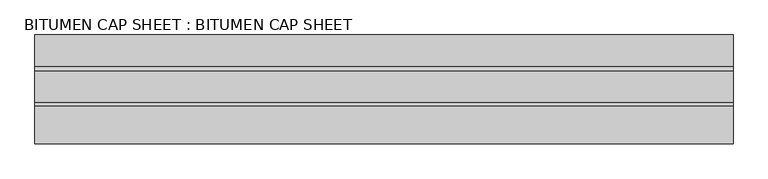
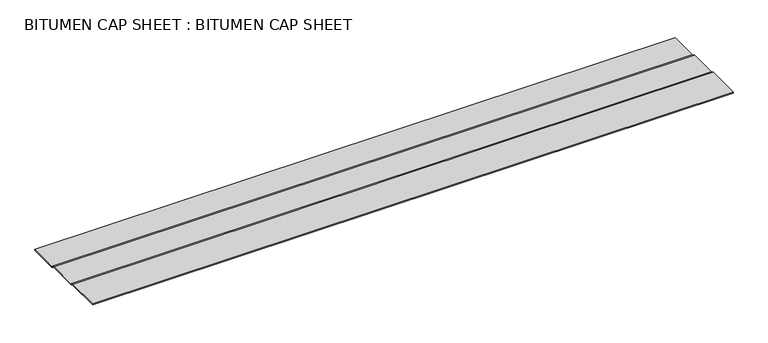
"""IFC4 building model written with IfcOpenShell, lengths in millimetres: proxy geometry, BITUMEN CAP SHEET : BITUMEN CAP SHEET."""

import ifcopenshell
import ifcopenshell.guid

model = None  # the IFC model being written
_history = None  # IfcOwnerHistory: only IFC2X3 demands one
_inside = {}  # id of a spatial element -> (the spatial element, [elements in it])
_under = {}  # id of a project, library or spatial element -> (it, [spatial elements below it])
_declared = {}  # id of a project -> (the project, [libraries it declares])
_typed = {}  # id of a type object -> (the type object, [elements of that type])
_made_of = {}  # id of a material, layer set ... -> (it, [elements and type objects made of it])


def new_model(schema):
    """Start an empty IFC model of exactly this schema.

    Asked for "IFC4X3", IfcOpenShell would pick the latest addendum, in which some entities
    have other attributes; the version numbers below select the first issue.
    IFC2X3 requires an IfcOwnerHistory on every rooted entity: one is made here for all.
    """
    global model, _history
    if schema == "IFC4X3":
        model = ifcopenshell.file(schema_version=(4, 3, 0, 0))
    else:
        model = ifcopenshell.file(schema=schema)
    _inside.clear()
    _under.clear()
    _declared.clear()
    _typed.clear()
    _made_of.clear()
    _history = None
    if model.schema == "IFC2X3":
        org = make("IfcOrganization", Name="unknown")
        user = make(
            "IfcPersonAndOrganization",
            ThePerson=make("IfcPerson", FamilyName="unknown"),
            TheOrganization=org,
        )
        app = make(
            "IfcApplication",
            ApplicationDeveloper=org,
            Version="unknown",
            ApplicationFullName="unknown",
            ApplicationIdentifier="unknown",
        )
        _history = make(
            "IfcOwnerHistory",
            OwningUser=user,
            OwningApplication=app,
            ChangeAction="ADDED",
            CreationDate=0,
        )
    return model


def make(cls, **values):
    """One entity of the class cls with the attributes given. An attribute that is None is left unset."""
    return model.create_entity(
        cls, **{name: value for name, value in values.items() if value is not None}
    )


def rooted(cls, **values):
    """An entity with a GlobalId (a new one), such as an element, a storey or a relation."""
    return make(cls, GlobalId=ifcopenshell.guid.new(), OwnerHistory=_history, **values)


def si_unit(unit_type, name, prefix=None):
    """IfcSIUnit, for example si_unit("LENGTHUNIT", "METRE", prefix="MILLI")."""
    return make("IfcSIUnit", UnitType=unit_type, Prefix=prefix, Name=name)


def assignment(units):
    """IfcUnitAssignment: the units of a project."""
    return None if units is None else make("IfcUnitAssignment", Units=units)


def point(xyz):
    """IfcCartesianPoint."""
    return None if xyz is None else make("IfcCartesianPoint", Coordinates=xyz)


def direction(xyz):
    """IfcDirection."""
    return None if xyz is None else make("IfcDirection", DirectionRatios=xyz)


def frame(location, z_axis=None, x_axis=None):
    """IfcAxis2Placement3D, a coordinate frame: its origin and axes. An axis left out is left unset."""
    return make(
        "IfcAxis2Placement3D",
        Location=point(location),
        Axis=direction(z_axis),
        RefDirection=direction(x_axis),
    )


def origin():
    """The frame at (0, 0, 0) with its axes left unset."""
    return frame((0.0, 0.0, 0.0))


def place(relative_to, where):
    """IfcLocalPlacement: puts the frame where relative to a parent placement (None: the world)."""
    return make(
        "IfcLocalPlacement", PlacementRelTo=relative_to, RelativePlacement=where
    )


def context(
    kind, dimensions, precision=None, world=None, true_north=None, identifier=None
):
    """IfcGeometricRepresentationContext, for example the 3D "Model" context."""
    return make(
        "IfcGeometricRepresentationContext",
        ContextIdentifier=identifier,
        ContextType=kind,
        CoordinateSpaceDimension=dimensions,
        Precision=precision,
        WorldCoordinateSystem=world,
        TrueNorth=true_north,
    )


def project(units=None, contexts=None):
    """IfcProject with its units and contexts."""
    return rooted(
        "IfcProject",
        Name="project",
        RepresentationContexts=contexts,
        UnitsInContext=assignment(units),
    )


def spatial(cls, under=None, at=None, **own):
    """A site, building, storey or space (cls), placed at a placement, below another one or the project."""
    s = rooted(cls, ObjectPlacement=at, **own)
    if under is not None:
        _under.setdefault(under.id(), (under, []))[1].append(s)
    return s


def polyline(points):
    """IfcPolyline through the points."""
    return make("IfcPolyline", Points=[point(p) for p in points])


def outline(outer, holes=None, kind="AREA"):
    """IfcArbitraryClosedProfileDef: a profile drawn as a closed curve; with holes, ...WithVoids."""
    if holes is None:
        return make("IfcArbitraryClosedProfileDef", ProfileType=kind, OuterCurve=outer)
    return make(
        "IfcArbitraryProfileDefWithVoids",
        ProfileType=kind,
        OuterCurve=outer,
        InnerCurves=holes,
    )


def extrude(swept, where, along, depth):
    """IfcExtrudedAreaSolid: the profile swept, set in the frame where, extruded along a direction by depth."""
    return make(
        "IfcExtrudedAreaSolid",
        SweptArea=swept,
        Position=where,
        ExtrudedDirection=direction(along),
        Depth=depth,
    )


def shape(context_of_items, identifier, shape_type, items):
    """IfcShapeRepresentation: the items that make up one representation, for example the "Body"."""
    return make(
        "IfcShapeRepresentation",
        ContextOfItems=context_of_items,
        RepresentationIdentifier=identifier,
        RepresentationType=shape_type,
        Items=items,
    )


def source(mapping_origin, context_of_items, identifier, shape_type, items):
    """IfcRepresentationMap: a shape defined once, which mapped items show again and again."""
    return make(
        "IfcRepresentationMap",
        MappingOrigin=mapping_origin,
        MappedRepresentation=shape(context_of_items, identifier, shape_type, items),
    )


def transform(
    local_origin,
    x_axis=None,
    y_axis=None,
    z_axis=None,
    scale=None,
    scale2=None,
    scale3=None,
    uniform=True,
):
    """IfcCartesianTransformationOperator3D, or its non-uniform kind. x_axis, y_axis, z_axis: its Axis1, 2, 3."""
    if uniform:
        return make(
            "IfcCartesianTransformationOperator3D",
            Axis1=direction(x_axis),
            Axis2=direction(y_axis),
            LocalOrigin=point(local_origin),
            Scale=scale,
            Axis3=direction(z_axis),
        )
    return make(
        "IfcCartesianTransformationOperator3DnonUniform",
        Axis1=direction(x_axis),
        Axis2=direction(y_axis),
        LocalOrigin=point(local_origin),
        Scale=scale,
        Axis3=direction(z_axis),
        Scale2=scale2,
        Scale3=scale3,
    )


def mapped(mapping_source, mapping_target):
    """IfcMappedItem: shows the shape of a source again, moved by a transform."""
    return make(
        "IfcMappedItem", MappingSource=mapping_source, MappingTarget=mapping_target
    )


def made_of(thing, what):
    """Note that an element or type object is made of a material, layer set ...; save() writes the relation."""
    if what is not None:
        _made_of.setdefault(what.id(), (what, []))[1].append(thing)
    return thing


def element(
    cls,
    number,
    at=None,
    inside=None,
    cuts=None,
    type_object=None,
    material=None,
    context=None,
    identifier="Body",
    shape_type=None,
    held_by="IfcProductDefinitionShape",
    body=None,
    shapes=None,
    **own,
):
    """One element of the class cls, such as IfcWall. Its Tag is "e" and its number.

    at: its placement. inside: the storey or other place that contains it. cuts: it is an
    opening in that element (IfcRelVoidsElement). A single representation is given by context,
    identifier, shape_type and body (its items); several are given by shapes. held_by: the class
    of the entity that holds the representations. save() writes the other relations.
    """
    e = rooted(cls, Tag="e%d" % number, ObjectPlacement=at, **own)
    if body is not None:
        shapes = [shape(context, identifier, shape_type, body)]
    if shapes is not None:
        e.Representation = make(held_by, Representations=shapes)
    if inside is not None:
        _inside.setdefault(inside.id(), (inside, []))[1].append(e)
    if cuts is not None:
        rooted(
            "IfcRelVoidsElement", RelatingBuildingElement=cuts, RelatedOpeningElement=e
        )
    if type_object is not None:
        _typed.setdefault(type_object.id(), (type_object, []))[1].append(e)
    return made_of(e, material)


def aggregate(whole, parts):
    """IfcRelAggregates: a whole, such as a stair, and the parts it consists of."""
    return rooted("IfcRelAggregates", RelatingObject=whole, RelatedObjects=parts)


def save(model, path):
    """Write the relations noted so far, then the file.

    IfcRelAggregates (storeys below a building ...), IfcRelContainedInSpatialStructure (elements
    in a storey), IfcRelDefinesByType, IfcRelAssociatesMaterial and IfcRelDeclares: one each for
    every whole, place, type object, material and project.
    """
    for whole, parts in _under.values():
        aggregate(whole, parts)
    for where, things in _inside.values():
        rooted(
            "IfcRelContainedInSpatialStructure",
            RelatedElements=things,
            RelatingStructure=where,
        )
    for kind, things in _typed.values():
        rooted("IfcRelDefinesByType", RelatedObjects=things, RelatingType=kind)
    for what, things in _made_of.values():
        rooted("IfcRelAssociatesMaterial", RelatedObjects=things, RelatingMaterial=what)
    for by, libraries in _declared.values():
        rooted("IfcRelDeclares", RelatingContext=by, RelatedDefinitions=libraries)
    model.write(path)


def bitumen_cap_sheet_bitumen_cap_sheet_a55ad838(model_context):
    return source(origin(), model_context, "Body", "SweptSolid", [
        extrude(outline(polyline([(-5237.2758356, 40238.7580714), (-5329.4404972, 40238.7580714), (-5341.9053158, 40244.0440809), (-5432.619472, 40244.0440809), (-5442.3358585, 40248.3766459), (-5549.5470696, 40248.3766459), (-5549.5470696, 40251.5518755), (-5441.660573, 40251.5518755), (-5431.9436715, 40247.2190809), (-5341.2599159, 40247.2190809), (-5328.7950972, 40241.9330714), (-5237.2758356, 40241.9330714), (-5237.2758356, 40238.7580714)])), frame((12382.7678845, 0.0, 0.0), z_axis=(1.0, 0.0, 0.0), x_axis=(0.0, 1.0, 0.0)), (0.0, 0.0, 1.0), 2000.25),
    ])


if __name__ == "__main__":
    model = new_model("IFC4")
    model_context = context("Model", 3, world=origin())
    ifc_project = project(units=[si_unit("LENGTHUNIT", "METRE", prefix="MILLI")], contexts=[model_context])
    site = spatial("IfcSite", under=ifc_project)
    building = spatial("IfcBuilding", under=site)
    placement = place(None, origin())
    bitumen_cap_sheet_bitumen_cap_sheet_shape = bitumen_cap_sheet_bitumen_cap_sheet_a55ad838(model_context)
    element("IfcBuildingElementProxy", 1, Name="BITUMEN CAP SHEET : BITUMEN CAP SHEET", ObjectType="BITUMEN CAP SHEET : BITUMEN CAP SHEET", at=placement, inside=building, context=model_context, shape_type="MappedRepresentation", body=[
        mapped(bitumen_cap_sheet_bitumen_cap_sheet_shape, transform((0.0, 0.0, 0.0), x_axis=(1.0, 0.0, 0.0), y_axis=(0.0, 1.0, 0.0), z_axis=(0.0, 0.0, 1.0))),
    ])
    save(model, "model.ifc")

# Revit data of these elements
# Type "BITUMEN CAP SHEET : BITUMEN CAP SHEET"
#   NameOverride = "BITUMEN CAP SHEET"
# Element 1 (IfcBuildingElementProxy, "BITUMEN CAP SHEET : BITUMEN CAP SHEET")
#   Materials on its faces: "MODIFIED BITUMEN GRANULE SURFACED CAP SHEET"
# Materials
#   "MODIFIED BITUMEN GRANULE SURFACED CAP SHEET": class "Unassigned", colour RGB 85 85 127, transparency 0
